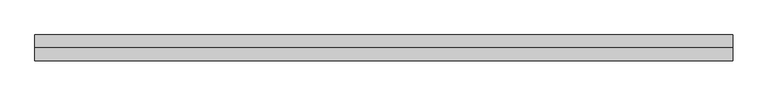
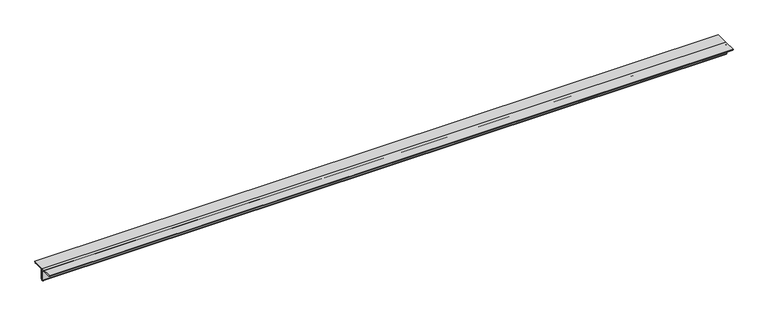
"""IFC4 building model written with IfcOpenShell, lengths in millimetres: member geometry, Steel Framing_2Ls_KS : H_SB_AR_S02_2Ls-100x100x10_VBR1."""

from ifc_helpers import new_model, si_unit, point, frame, frame_2d, origin, place, context, project, spatial, polyline, circle_curve, trimmed, segment, composite_curve, outline, extrude, source, transform, mapped, element, save


def member_2ba16a47(model_context):
    return source(origin(), model_context, "Body", "SweptSolid", [
        extrude(outline(composite_curve([segment(polyline([(0.0, 28.2), (0.0, -71.8)]), True, "CONTINUOUS"), segment(trimmed(circle_curve(frame_2d((0.0, -61.8)), 10.0), [point((0.0, -71.8))], [point((-10.0, -61.8))], False, "CARTESIAN"), True, "CONTINUOUS"), segment(polyline([(-10.0, -61.8), (-10.0, 8.2)]), True, "CONTINUOUS"), segment(trimmed(circle_curve(frame_2d((-20.0, 8.2)), 10.0), [point((-10.0, 8.2))], [point((-20.0, 18.2))], True, "CARTESIAN"), True, "CONTINUOUS"), segment(polyline([(-20.0, 18.2), (-90.0, 18.2)]), True, "CONTINUOUS"), segment(trimmed(circle_curve(frame_2d((-90.0, 28.2)), 10.0), [point((-90.0, 18.2))], [point((-100.0, 28.2))], False, "CARTESIAN"), True, "CONTINUOUS"), segment(polyline([(-100.0, 28.2), (0.0, 28.2)]), True, "CONTINUOUS")], self_intersect=False)), frame((-2634.5127122, 0.0, 0.0), z_axis=(1.0, 0.0, 0.0), x_axis=(0.0, 1.0, 0.0)), (0.0, 0.0, 1.0), 5399.8099488),
        extrude(outline(composite_curve([segment(polyline([(0.0, 28.2), (100.0, 28.2)]), True, "CONTINUOUS"), segment(trimmed(circle_curve(frame_2d((90.0, 28.2)), 10.0), [point((100.0, 28.2))], [point((90.0, 18.2))], False, "CARTESIAN"), True, "CONTINUOUS"), segment(polyline([(90.0, 18.2), (20.0, 18.2)]), True, "CONTINUOUS"), segment(trimmed(circle_curve(frame_2d((20.0, 8.2)), 10.0), [point((20.0, 18.2))], [point((10.0, 8.2))], True, "CARTESIAN"), True, "CONTINUOUS"), segment(polyline([(10.0, 8.2), (10.0, -61.8)]), True, "CONTINUOUS"), segment(trimmed(circle_curve(frame_2d((0.0, -61.8)), 10.0), [point((10.0, -61.8))], [point((0.0, -71.8))], False, "CARTESIAN"), True, "CONTINUOUS"), segment(polyline([(0.0, -71.8), (0.0, 28.2)]), True, "CONTINUOUS")], self_intersect=False)), frame((-2634.5127122, 0.0, 0.0), z_axis=(1.0, 0.0, 0.0), x_axis=(0.0, 1.0, 0.0)), (0.0, 0.0, 1.0), 5399.8099488),
    ])


if __name__ == "__main__":
    model = new_model("IFC4")
    model_context = context("Model", 3, world=origin())
    ifc_project = project(units=[si_unit("LENGTHUNIT", "METRE", prefix="MILLI")], contexts=[model_context])
    site = spatial("IfcSite", under=ifc_project)
    building = spatial("IfcBuilding", under=site)
    placement = place(None, origin())
    member_shape = member_2ba16a47(model_context)
    element("IfcMember", 1, ObjectType="Steel Framing_2Ls_KS : H_SB_AR_S02_2Ls-100x100x10_VBR1", at=placement, inside=building, context=model_context, shape_type="MappedRepresentation", body=[
        mapped(member_shape, transform((0.0, 0.0, 0.0), x_axis=(1.0, 0.0, 0.0), y_axis=(0.0, 1.0, 0.0), z_axis=(0.0, 0.0, 1.0))),
    ])
    save(model, "model.ifc")

# Revit data of these elements
# Type "Steel Framing_2Ls_KS : H_SB_AR_S02_2Ls-100x100x10_VBR1"
#   Type Comments = "MAIN"
#   Type Mark = "VBR1"
#   H_SectionID = "2Ls-100x100x10"
#   Assembly Code = "B10"
#   Legs = "LLBB"
#   H_Ratio for Additional Steel Plate = 0.2
#   W = 0
#   Perimeter = 0.80 m²/m
#   Nominal Weight = 29.80 kgf/m
#   Length [instance default] = 1524 mm
#   Space = 0 mm
#   b = 100 mm
#   d = 100 mm
#   t = 10 mm
#   y = 28.2 mm
#   A = 0.0038 m²
#   Structural Material [instance default] = Steel, 45-345
# Element 1 (IfcMember, "Steel Framing_2Ls_KS : H_SB_AR_S02_2Ls-100x100x10_VBR1")
#   Materials on its faces: "Steel, 45-345"
# Materials
#   "Steel, 45-345": class "Metal", colour RGB 189 187 185, transparency 0, Description = "Steel 345 MPa", Cost = 0
